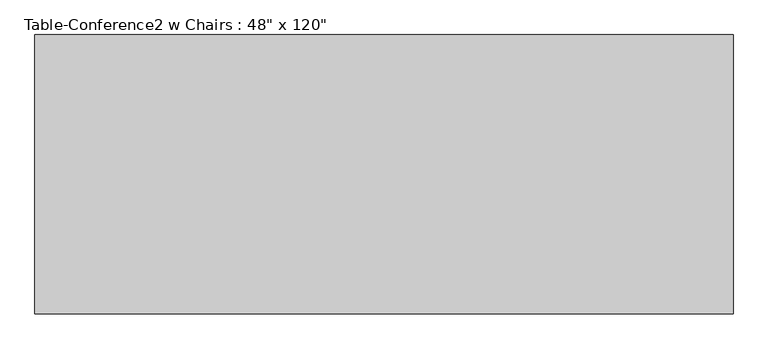
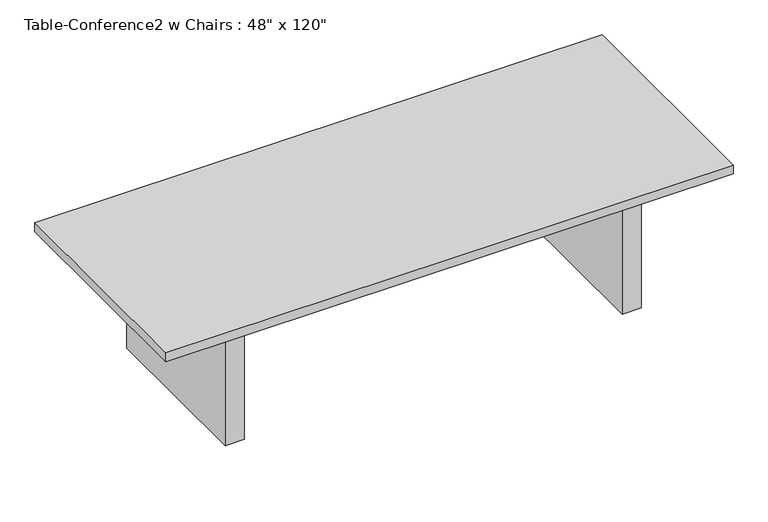
"""IFC4 building model written with IfcOpenShell, lengths in millimetres: furniture geometry."""

from ifc_helpers import new_model, si_unit, frame, origin, origin_with_axes, place, context, project, spatial, polyline, outline, extrude, source, transform, mapped, element, save


def furniture_098dae9e(model_context):
    return source(origin(), model_context, "Body", "SweptSolid", [
        extrude(outline(polyline([(1016.0, 457.2), (1016.0, 419.1), (-1016.0, 419.1), (-1016.0, 457.2), (1016.0, 457.2)])), frame((0.0, 0.0, 609.6), z_axis=(0.0, 0.0, 1.0), x_axis=(1.0, 0.0, 0.0)), (0.0, 0.0, 1.0), 101.6),
        extrude(outline(polyline([(1016.0, -457.2), (-1016.0, -457.2), (-1016.0, -419.1), (1016.0, -419.1), (1016.0, -457.2)])), frame((0.0, 0.0, 609.6), z_axis=(0.0, 0.0, 1.0), x_axis=(1.0, 0.0, 0.0)), (0.0, 0.0, 1.0), 101.6),
        extrude(outline(polyline([(-1016.0, -457.2), (-1117.6, -457.2), (-1117.6, 457.2), (-1016.0, 457.2), (-1016.0, -457.2)])), origin_with_axes(), (0.0, 0.0, 1.0), 711.2),
        extrude(outline(polyline([(1117.6, -457.2), (1016.0, -457.2), (1016.0, 457.2), (1117.6, 457.2), (1117.6, -457.2)])), origin_with_axes(), (0.0, 0.0, 1.0), 711.2),
        extrude(outline(polyline([(1524.0, -609.6), (-1524.0, -609.6), (-1524.0, 609.6), (1524.0, 609.6), (1524.0, -609.6)])), frame((0.0, 0.0, 711.2), z_axis=(0.0, 0.0, 1.0), x_axis=(1.0, 0.0, 0.0)), (0.0, 0.0, 1.0), 50.8),
    ])


if __name__ == "__main__":
    model = new_model("IFC4")
    model_context = context("Model", 3, world=origin())
    ifc_project = project(units=[si_unit("LENGTHUNIT", "METRE", prefix="MILLI")], contexts=[model_context])
    site = spatial("IfcSite", under=ifc_project)
    building = spatial("IfcBuilding", under=site)
    placement = place(None, origin())
    furniture_shape = furniture_098dae9e(model_context)
    element("IfcFurniture", 1, ObjectType="Table-Conference2 w Chairs : 48\" x 120\"", at=placement, inside=building, context=model_context, shape_type="MappedRepresentation", body=[
        mapped(furniture_shape, transform((0.0, 0.0, 0.0), x_axis=(1.0, 0.0, 0.0), y_axis=(0.0, 1.0, 0.0), z_axis=(0.0, 0.0, 1.0))),
    ])
    save(model, "model.ifc")

# Revit data of these elements
# Project information
#   Projekt-Nummer = "Hier die Projektnummer eintragen!"
#   IfcSite GUID = "3DdyCULLv3kQRx$MQ8PThJ"
#   IfcBuilding GUID = "3DdyCULLv3kQRx$MQ8PThG"
#   IfcProject GUID = "3DdyCULLv3kQRx$MQ8PThH"
#   Classification.Facility.Number = "Co_20_15_58"
#   Classification.Facility.Description = "Office complexes"
#   Project Status = "Projektstatus"
#   Project Address = "Geben Sie die Adresse hier ein"
# Type "Table-Conference2 w Chairs : 48\" x 120\""
#   Type IfcGUID = "2u0XNFrAPALBFZCv81fqig"
#   Assembly Code = "E2020200"
#   Description = "Seating 10-12"
#   Height = 0.762 m
#   Length = 3.048 m
#   Width = 1.2192 m
#   Number Of Chairs One Side = 4
#   Number Of Chairs = 10
#   Material = Wood - Cherry
#   Default Elevation = 0
# Element 1 (IfcFurniture, "Table-Conference2 w Chairs : 48\" x 120\"")
#   Materials on its faces: "Wood - Cherry"
# Materials
#   "Wood - Cherry": class "Wood", colour RGB 226 177 128, transparency 0
